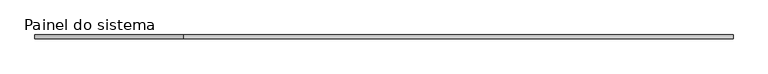
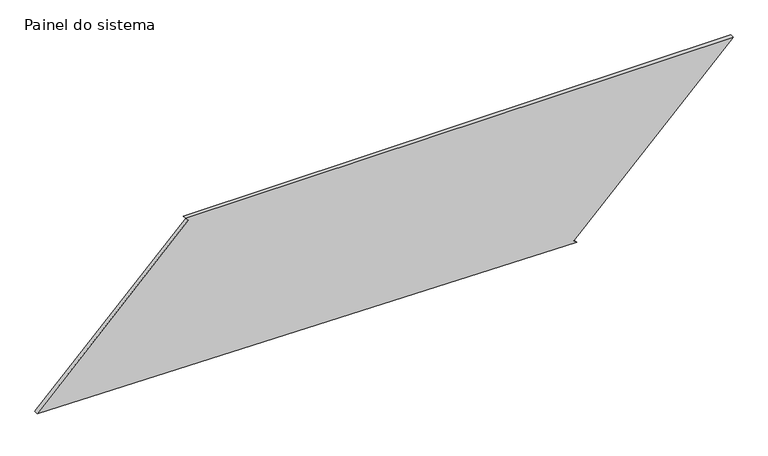
"""IFC4 building model written with IfcOpenShell, lengths in millimetres: plate geometry, Painel do sistema : Envidraçado."""

from ifc_helpers import new_model, si_unit, frame, origin, place, context, project, spatial, polyline, outline, extrude, source, transform, mapped, element, save


def painel_do_sistema_e2001369(model_context):
    return source(origin(), model_context, "Body", "SweptSolid", [
        extrude(outline(polyline([(0.0, 1258.9494237), (17.655268, 1241.249381), (1066.4600258, 2287.4010464), (1066.4600258, -1310.9362368), (1048.8047577, -1293.2361942), (52.1186543, -2287.4010464), (0.0, 1258.9494237)])), frame((0.0, 24.5, 0.0), z_axis=(0.0, 1.0, 0.0), x_axis=(0.0, 0.0, 1.0)), (0.0, 0.0, 1.0), 25.0),
    ])


if __name__ == "__main__":
    model = new_model("IFC4")
    model_context = context("Model", 3, world=origin())
    ifc_project = project(units=[si_unit("LENGTHUNIT", "METRE", prefix="MILLI")], contexts=[model_context])
    site = spatial("IfcSite", under=ifc_project)
    building = spatial("IfcBuilding", under=site)
    placement = place(None, origin())
    painel_do_sistema_shape = painel_do_sistema_e2001369(model_context)
    element("IfcPlate", 1, ObjectType="Painel do sistema : Envidraçado", at=placement, inside=building, context=model_context, shape_type="MappedRepresentation", body=[
        mapped(painel_do_sistema_shape, transform((0.0, 0.0, 0.0), x_axis=(1.0, 0.0, 0.0), y_axis=(0.0, 1.0, 0.0), z_axis=(0.0, 0.0, 1.0))),
    ])
    save(model, "model.ifc")

# Revit data of these elements
# Type "Painel do sistema : Envidraçado"
#   Construction Type Id = "GSP4R"
#   Analytic Construction = "Vidraça única Pilkington 1/8 pol"
#   Visual Light Transmittance = 0.9
#   Solar Heat Gain Coefficient = 0.86
#   Heat Transfer Coefficient (U) = 6.7069 W/(m²·K)
# Element 1 (IfcPlate, "Painel do sistema : Envidraçado")
#   Materials on its faces: "Vidro"
# Materials
#   "Vidro": class "Vidro", colour RGB 0 128 192, transparency 0.9, Description = "Vidro de sílica", Cost = 0
